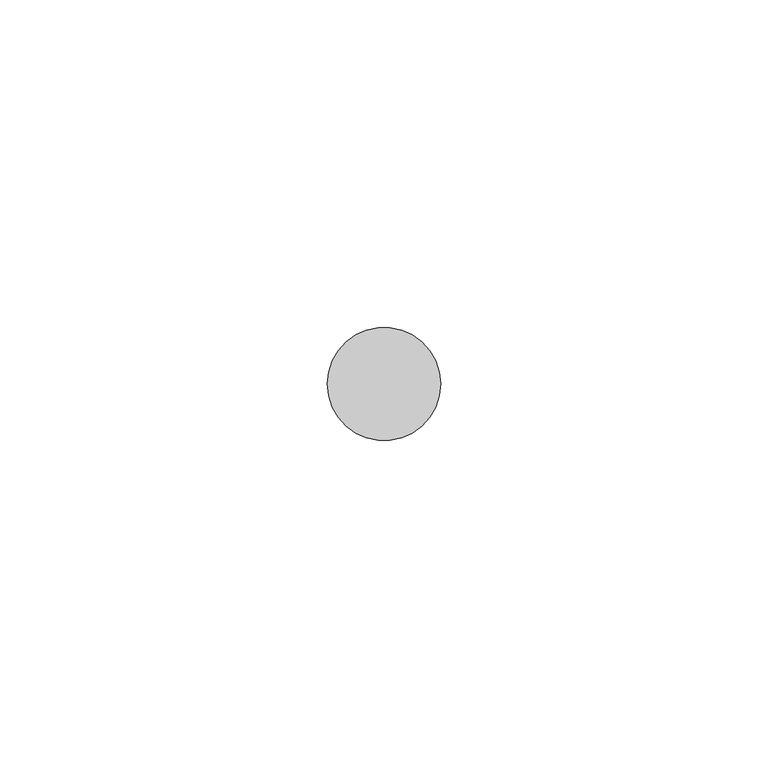
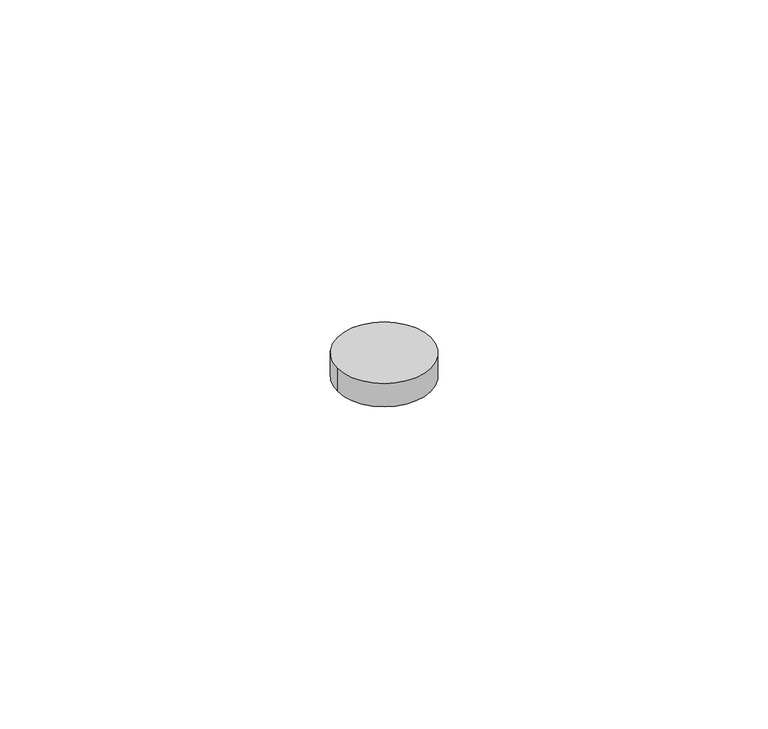
"""IFC4 building model written with IfcOpenShell, lengths in millimetres: proxy geometry, Hinge Pin Keeper7 : Hinge Pin Keeper."""

from ifc_helpers import new_model, si_unit, point, frame, frame_2d, origin, place, context, project, spatial, circle_curve, trimmed, segment, composite_curve, outline, extrude, source, transform, mapped, element, save


def generic_models_10b8f884(model_context):
    return source(origin(), model_context, "Body", "SweptSolid", [
        extrude(outline(composite_curve([segment(trimmed(circle_curve(frame_2d((587319.1320739, -534100.7049841)), 8.6534625), [point((587310.4786114, -534100.7049841))], [point((587327.7855364, -534100.7049841))], False, "CARTESIAN"), True, "CONTINUOUS"), segment(trimmed(circle_curve(frame_2d((587319.1320739, -534100.7049841)), 8.6534625), [point((587327.7855364, -534100.7049841))], [point((587310.4786114, -534100.7049841))], False, "CARTESIAN"), True, "CONTINUOUS")], self_intersect=False)), frame((0.0, 0.0, 2084.5859375), z_axis=(0.0, 0.0, 1.0), x_axis=(1.0, 0.0, 0.0)), (0.0, 0.0, 1.0), 4.5640625),
    ])


if __name__ == "__main__":
    model = new_model("IFC4")
    model_context = context("Model", 3, world=origin())
    ifc_project = project(units=[si_unit("LENGTHUNIT", "METRE", prefix="MILLI")], contexts=[model_context])
    site = spatial("IfcSite", under=ifc_project)
    building = spatial("IfcBuilding", under=site)
    placement = place(None, origin())
    generic_models_shape = generic_models_10b8f884(model_context)
    element("IfcBuildingElementProxy", 1, Name="Hinge Pin Keeper7 : Hinge Pin Keeper", ObjectType="Hinge Pin Keeper7 : Hinge Pin Keeper", at=placement, inside=building, context=model_context, shape_type="MappedRepresentation", body=[
        mapped(generic_models_shape, transform((0.0, 0.0, 0.0), x_axis=(1.0, 0.0, 0.0), y_axis=(0.0, 1.0, 0.0), z_axis=(0.0, 0.0, 1.0))),
    ])
    save(model, "model.ifc")

# Revit data of these elements
# Element 1 (IfcBuildingElementProxy, "Hinge Pin Keeper7 : Hinge Pin Keeper")
#   Materials on its faces: "6\"X6\" WELD-ON STL BUTT HINGE"
# Materials
#   "6\"X6\" WELD-ON STL BUTT HINGE": class "Metal", colour RGB 189 187 185, transparency 0, Description = "Carbon steel", Cost = 0
